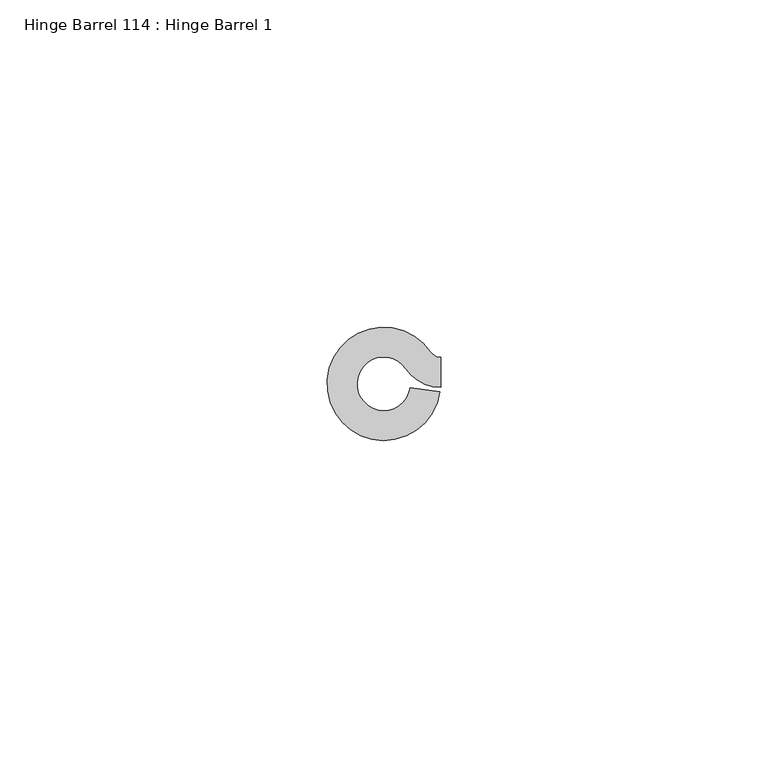
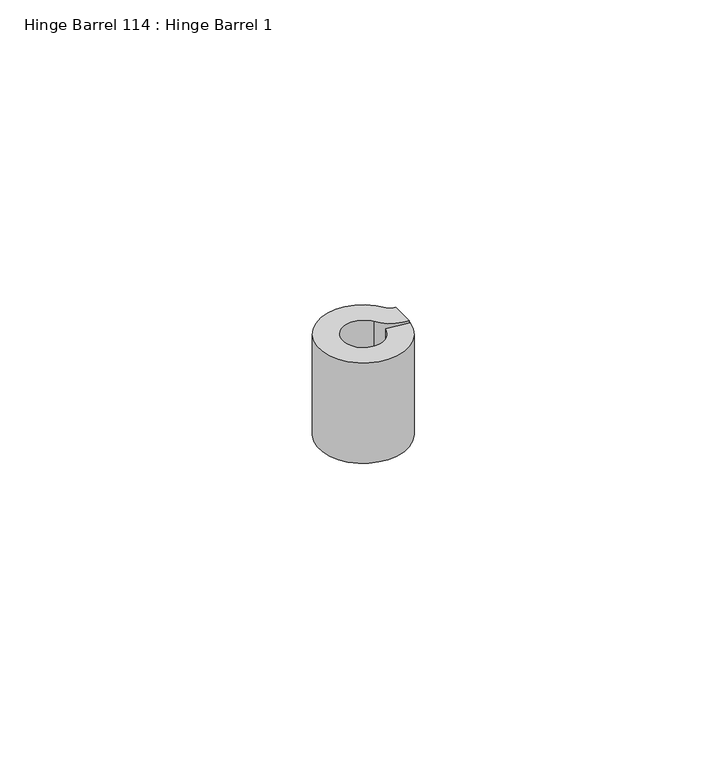
"""IFC4 building model written with IfcOpenShell, lengths in millimetres: proxy geometry, Hinge Barrel 114 : Hinge Barrel 1."""

from ifc_helpers import new_model, si_unit, point, frame, frame_2d, origin, place, context, project, spatial, polyline, circle_curve, trimmed, segment, composite_curve, outline, extrude, source, transform, mapped, element, save


def hinge_barrel_114_hinge_barrel_1_1e33f8db(model_context):
    return source(origin(), model_context, "Body", "SweptSolid", [
        extrude(outline(composite_curve([segment(trimmed(circle_curve(frame_2d((587319.1320739, -534100.7049841)), 4.0894), [point((587322.5194669, -534098.4139665))], [point((587323.1821338, -534101.2708529))], True, "CARTESIAN"), True, "CONTINUOUS"), segment(polyline([(587323.1821338, -534101.2708529), (587327.7022899, -534101.9024028)]), True, "CONTINUOUS"), segment(trimmed(circle_curve(frame_2d((587319.1320739, -534100.7049841)), 8.6534625), [point((587327.7022899, -534101.9024028))], [point((587326.3000393, -534095.8570273))], False, "CARTESIAN"), True, "CONTINUOUS"), segment(trimmed(circle_curve(frame_2d((587327.8245257, -534094.8259615)), 1.8404226), [point((587326.3000393, -534095.8570273))], [point((587327.8245257, -534096.6663841))], True, "CARTESIAN"), True, "CONTINUOUS"), segment(polyline([(587327.8245257, -534096.6663841), (587327.8245257, -534101.2304466)]), True, "CONTINUOUS"), segment(trimmed(circle_curve(frame_2d((587327.8245257, -534094.8259615)), 6.4044851), [point((587327.8245257, -534101.2304466))], [point((587322.5194669, -534098.4139665))], False, "CARTESIAN"), True, "CONTINUOUS")], self_intersect=False)), frame((0.0, 0.0, 438.15), z_axis=(0.0, 0.0, 1.0), x_axis=(1.0, 0.0, 0.0)), (0.0, 0.0, 1.0), 20.8359375),
    ])


if __name__ == "__main__":
    model = new_model("IFC4")
    model_context = context("Model", 3, world=origin())
    ifc_project = project(units=[si_unit("LENGTHUNIT", "METRE", prefix="MILLI")], contexts=[model_context])
    site = spatial("IfcSite", under=ifc_project)
    building = spatial("IfcBuilding", under=site)
    placement = place(None, origin())
    hinge_barrel_114_hinge_barrel_1_shape = hinge_barrel_114_hinge_barrel_1_1e33f8db(model_context)
    element("IfcBuildingElementProxy", 1, Name="Hinge Barrel 114 : Hinge Barrel 1", ObjectType="Hinge Barrel 114 : Hinge Barrel 1", at=placement, inside=building, context=model_context, shape_type="MappedRepresentation", body=[
        mapped(hinge_barrel_114_hinge_barrel_1_shape, transform((0.0, 0.0, 0.0), x_axis=(1.0, 0.0, 0.0), y_axis=(0.0, 1.0, 0.0), z_axis=(0.0, 0.0, 1.0))),
    ])
    save(model, "model.ifc")

# Revit data of these elements
# Element 1 (IfcBuildingElementProxy, "Hinge Barrel 114 : Hinge Barrel 1")
#   Materials on its faces: "6\"X6\" WELD-ON STL BUTT HINGE"
# Materials
#   "6\"X6\" WELD-ON STL BUTT HINGE": class "Metal", colour RGB 189 187 185, transparency 0, Description = "Carbon steel", Cost = 0
